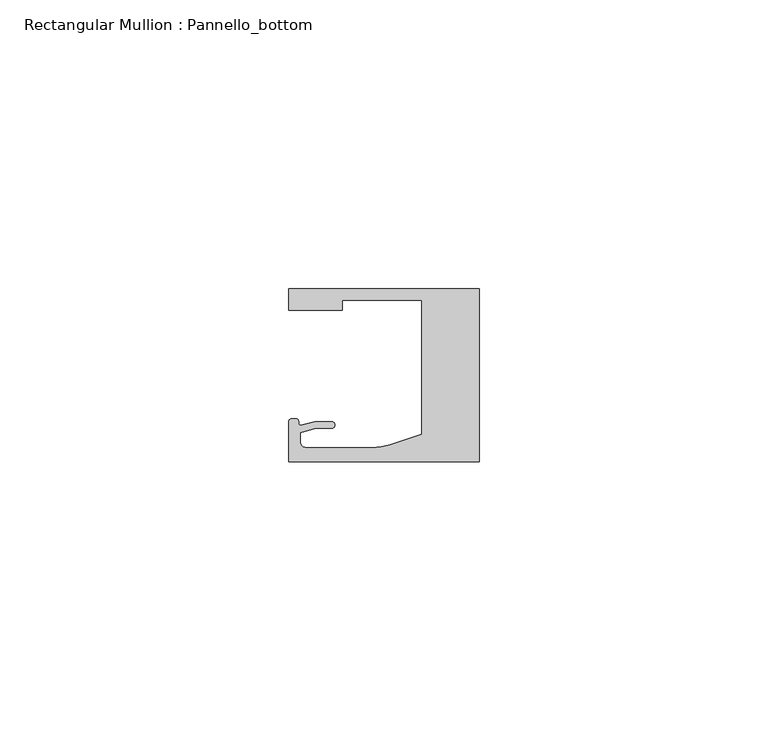
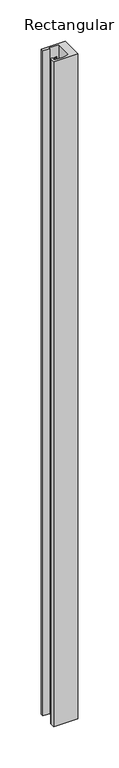
"""IFC4 building model written with IfcOpenShell, lengths in millimetres: member geometry, Rectangular Mullion : Pannello_bottom."""

from ifc_helpers import new_model, si_unit, frame, origin, place, context, project, spatial, polyline, circle_curve, source, transform, mapped, element, save
from ifc_brep_helpers import plane_surface, cylinder_surface, revolved_surface, extruded_surface, spline_curve, advanced_brep


def rectangular_mullion_pannello_bottom_af961b8c(model_context):
    return source(origin(), model_context, "Body", "AdvancedBrep", [
        advanced_brep(
        [(-33.0, 15.0, 0.0), (-33.0, 11.3000004, 0.0), (-23.700041, 11.3000004, 0.0), (-23.700041, 13.0000004, 0.0), (-9.9999723, 13.0000004, 0.0), (-9.9999723, -10.2367227, 0.0), (-15.4591336, -12.0105099, 0.0), (-18.5493024, -12.4999438, 0.0), (-30.0000002, -12.4999419, 0.0), (-31.0, -11.4999419, 0.0), (-31.0, -9.9121746, 0.0), (-28.3419477, -9.1999523, 0.0), (-25.59998, -9.1999523, 0.0), (-25.59998, -7.9999523, 0.0), (-28.4999305, -7.9999523, 0.0), (-30.9223017, -8.6490241, 0.0), (-33.0000135, -8.0000472, 0.0), (-33.0000135, -15.0, 0.0), (0.0, -15.0, 0.0), (0.0, 15.0, 0.0), (-33.0, 15.0, -980.0), (0.0, 15.0, -980.0), (0.0, -15.0, -980.0), (-33.0000135, -15.0, -980.0), (-33.0000135, -8.0000472, -980.0), (-30.9223017, -8.6490241, -980.0), (-28.4999305, -7.9999523, -980.0), (-25.59998, -7.9999523, -980.0), (-25.59998, -9.1999523, -980.0), (-28.3419477, -9.1999523, -980.0), (-31.0, -9.9121746, -980.0), (-31.0, -11.4999419, -980.0), (-30.0000002, -12.4999419, -980.0), (-18.5493024, -12.4999438, -980.0), (-15.4591336, -12.0105099, -980.0), (-9.9999723, -10.2367227, -980.0), (-9.9999723, 13.0000004, -980.0), (-23.700041, 13.0000004, -980.0), (-23.700041, 11.3000004, -980.0), (-33.0, 11.3000004, -980.0)],
        [
            (0, 1),
            (1, 2),
            (2, 3),
            (3, 4),
            (4, 5),
            (5, 6),
            (6, 7, circle_curve(frame((-18.5493007, -2.4999438, 0.0), z_axis=(0.0, 0.0, -1.0), x_axis=(0.0, -1.0, 0.0)), 10.0)),
            (7, 8),
            (8, 9, circle_curve(frame((-30.0, -11.4999419, 0.0), z_axis=(0.0, 0.0, -1.0), x_axis=(0.0, -1.0, 0.0)), 1.0)),
            (9, 10),
            (10, 11),
            (11, 12),
            (12, 13, circle_curve(frame((-25.59998, -8.5999523, 0.0), z_axis=(0.0, 0.0, 1.0), x_axis=(0.0, -1.0, 0.0)), 0.6)),
            (13, 14),
            (14, 15),
            (15, 16, spline_curve(3, [(-30.9223017, -8.6490241, 0.0), (-31.312054066, -8.717747958, 0.0), (-31.298563602, -8.366228555, 0.0), (-31.305645054, -7.690065204, 0.0), (-31.357433266, -7.563996614, 0.0), (-32.262327879, -7.456527435, 0.0), (-33.0000135, -7.457047519, 0.0), (-33.0000135, -8.0000472, 0.0)], [4, 2, 2, 4], [0.0, 0.001840817752199412, 0.004996616814974408, 0.007702013405570312])),
            (16, 17),
            (17, 18),
            (18, 19),
            (19, 0),
            (20, 21),
            (21, 22),
            (22, 23),
            (23, 24),
            (24, 25, spline_curve(3, [(-33.0000135, -8.0000472, -980.0), (-33.0000135, -7.457047519, -980.0), (-32.262327879, -7.456527435, -980.0), (-31.357433266, -7.563996614, -980.0), (-31.305645054, -7.690065204, -980.0), (-31.298563602, -8.366228555, -980.0), (-31.312054066, -8.717747958, -980.0), (-30.9223017, -8.6490241, -980.0)], [4, 2, 2, 4], [0.0, 0.0027053965905959043, 0.0058611956533709, 0.007702013405570312])),
            (25, 26),
            (26, 27),
            (27, 28, circle_curve(frame((-25.59998, -8.5999523, -980.0), z_axis=(0.0, 0.0, -1.0), x_axis=(0.0, -1.0, 0.0)), 0.6)),
            (28, 29),
            (29, 30),
            (30, 31),
            (31, 32, circle_curve(frame((-30.0, -11.4999419, -980.0), z_axis=(0.0, 0.0, 1.0), x_axis=(0.0, -1.0, 0.0)), 1.0)),
            (32, 33),
            (33, 34, circle_curve(frame((-18.5493007, -2.4999438, -980.0), z_axis=(0.0, 0.0, 1.0), x_axis=(0.0, -1.0, 0.0)), 10.0)),
            (34, 35),
            (35, 36),
            (36, 37),
            (37, 38),
            (38, 39),
            (39, 20),
            (0, 20),
            (39, 1),
            (38, 2),
            (37, 3),
            (36, 4),
            (35, 5),
            (34, 6),
            (33, 7),
            (32, 8),
            (31, 9),
            (30, 10),
            (29, 11),
            (28, 12),
            (27, 13),
            (26, 14),
            (25, 15),
            (24, 16),
            (23, 17),
            (22, 18),
            (21, 19),
        ],
        [
            plane_surface(frame((0.0, -36.2491502, 0.0), z_axis=(0.0, 0.0, 1.0), x_axis=(-1.0, 0.0, 0.0))),
            plane_surface(frame((0.0, -36.2491502, -980.0), z_axis=(0.0, 0.0, -1.0), x_axis=(-1.0, 0.0, 0.0))),
            plane_surface(frame((-33.0, 15.0, 0.0), z_axis=(-1.0, 0.0, 0.0), x_axis=(0.0, 0.0, -1.0))),
            plane_surface(frame((-33.0, 11.3000004, 0.0), z_axis=(0.0, -1.0, 0.0), x_axis=(0.0, 0.0, -1.0))),
            plane_surface(frame((-23.700041, 11.3000004, 0.0), z_axis=(1.0, 0.0, 0.0), x_axis=(0.0, 0.0, -1.0))),
            plane_surface(frame((-23.700041, 13.0000004, 0.0), z_axis=(0.0, -1.0, 0.0), x_axis=(0.0, 0.0, -1.0))),
            plane_surface(frame((-9.9999723, 13.0000004, 0.0), z_axis=(-1.0, 0.0, 0.0), x_axis=(0.0, 0.0, -1.0))),
            plane_surface(frame((-9.9999723, -10.2367227, 0.0), z_axis=(-0.30901670911956314, 0.9510566089801992, 0.0), x_axis=(0.0, 0.0, -1.0))),
            revolved_surface(polyline([(-18.5493007, -12.4999438, -980.0), (-18.5493007, -12.4999438, 0.0)]), (-18.5493007, -2.4999438, 0.0), (0.0, 0.0, -1.0)),
            plane_surface(frame((-18.5493024, -12.4999438, 0.0), z_axis=(1.6923026533778639e-07, 0.9999999999999858, 0.0), x_axis=(0.0, 0.0, -1.0))),
            revolved_surface(polyline([(-30.0, -12.4999419, -980.0), (-30.0, -12.4999419, 0.0)]), (-30.0, -11.4999419, 0.0), (0.0, 0.0, -1.0)),
            plane_surface(frame((-31.0, -11.4999419, 0.0), z_axis=(1.0, 0.0, 0.0), x_axis=(0.0, 0.0, -1.0))),
            plane_surface(frame((-31.0, -9.9121746, 0.0), z_axis=(0.25881883204288636, -0.9659258833782002, 0.0), x_axis=(0.0, 0.0, -1.0))),
            plane_surface(frame((-28.3419477, -9.1999523, 0.0), z_axis=(0.0, -1.0, 0.0), x_axis=(0.0, 0.0, -1.0))),
            cylinder_surface(frame((-25.59998, -8.5999523, 0.0), z_axis=(0.0, 0.0, 1.0), x_axis=(0.0, -1.0, 0.0)), 0.6),
            plane_surface(frame((-25.59998, -7.9999523, 0.0), z_axis=(0.0, 1.0, 0.0), x_axis=(0.0, 0.0, -1.0))),
            plane_surface(frame((-28.4999305, -7.9999523, 0.0), z_axis=(-0.25881883200192934, 0.9659258833891746, 0.0), x_axis=(0.0, 0.0, -1.0))),
            extruded_surface(spline_curve(3, [(-30.9223017, -8.6490241, -980.0), (-31.312054066, -8.717747958, -980.0), (-31.298563602, -8.366228555, -980.0), (-31.305645054, -7.690065204, -980.0), (-31.357433266, -7.563996614, -980.0), (-32.262327879, -7.456527435, -980.0), (-33.0000135, -7.457047519, -980.0), (-33.0000135, -8.0000472, -980.0)], [4, 2, 2, 4], [0.0, 0.001840817752199412, 0.004996616814974408, 0.007702013405570312]), (0.0, 0.0, 980.0), 980.0),
            plane_surface(frame((-33.0000135, -8.0000472, 0.0), z_axis=(-1.0, 0.0, 0.0), x_axis=(0.0, 0.0, -1.0))),
            plane_surface(frame((-33.0000135, -15.0, 0.0), z_axis=(0.0, -1.0, 0.0), x_axis=(0.0, 0.0, -1.0))),
            plane_surface(frame((0.0, -15.0, 0.0), z_axis=(1.0, 0.0, 0.0), x_axis=(0.0, 0.0, -1.0))),
            plane_surface(frame((0.0, 15.0, 0.0), z_axis=(0.0, 1.0, 0.0), x_axis=(0.0, 0.0, -1.0))),
        ],
        [
            (0, [[1, 2, 3, 4, 5, 6, 7, 8, 9, 10, 11, 12, 13, 14, 15, 16, 17, 18, 19, 20]]),
            (1, [[21, 22, 23, 24, 25, 26, 27, 28, 29, 30, 31, 32, 33, 34, 35, 36, 37, 38, 39, 40]]),
            (2, [[-1, 41, -40, 42]]),
            (3, [[-2, -42, -39, 43]]),
            (4, [[-3, -43, -38, 44]]),
            (5, [[-4, -44, -37, 45]]),
            (6, [[-5, -45, -36, 46]]),
            (7, [[-6, -46, -35, 47]]),
            (8, [[-7, -47, -34, 48]]),
            (9, [[-8, -48, -33, 49]]),
            (10, [[-9, -49, -32, 50]]),
            (11, [[-10, -50, -31, 51]]),
            (12, [[-11, -51, -30, 52]]),
            (13, [[-12, -52, -29, 53]]),
            (14, [[-13, -53, -28, 54]]),
            (15, [[-14, -54, -27, 55]]),
            (16, [[-15, -55, -26, 56]]),
            (17, [[-16, -56, -25, 57]]),
            (18, [[-17, -57, -24, 58]]),
            (19, [[-18, -58, -23, 59]]),
            (20, [[-19, -59, -22, 60]]),
            (21, [[-20, -60, -21, -41]]),
        ],
    ),
    ])


if __name__ == "__main__":
    model = new_model("IFC4")
    model_context = context("Model", 3, world=origin())
    ifc_project = project(units=[si_unit("LENGTHUNIT", "METRE", prefix="MILLI")], contexts=[model_context])
    site = spatial("IfcSite", under=ifc_project)
    building = spatial("IfcBuilding", under=site)
    placement = place(None, origin())
    rectangular_mullion_pannello_bottom_shape = rectangular_mullion_pannello_bottom_af961b8c(model_context)
    element("IfcMember", 1, ObjectType="Rectangular Mullion : Pannello_bottom", at=placement, inside=building, context=model_context, shape_type="MappedRepresentation", body=[
        mapped(rectangular_mullion_pannello_bottom_shape, transform((0.0, 0.0, 0.0), x_axis=(1.0, 0.0, 0.0), y_axis=(0.0, 1.0, 0.0), z_axis=(0.0, 0.0, 1.0))),
    ])
    save(model, "model.ifc")

# Revit data of these elements
# Type "Rectangular Mullion : Pannello_bottom"
#   built-in parameter 1007322 = 0.0984252 (stored number, unit not read)
#   built-in parameter 1007321 = 0.0328083 (stored number, unit not read)
#   built-in parameter 1007320 = 0 (stored number, unit not read)
